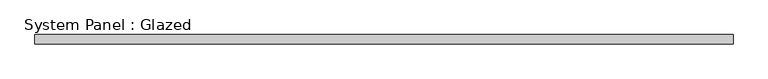
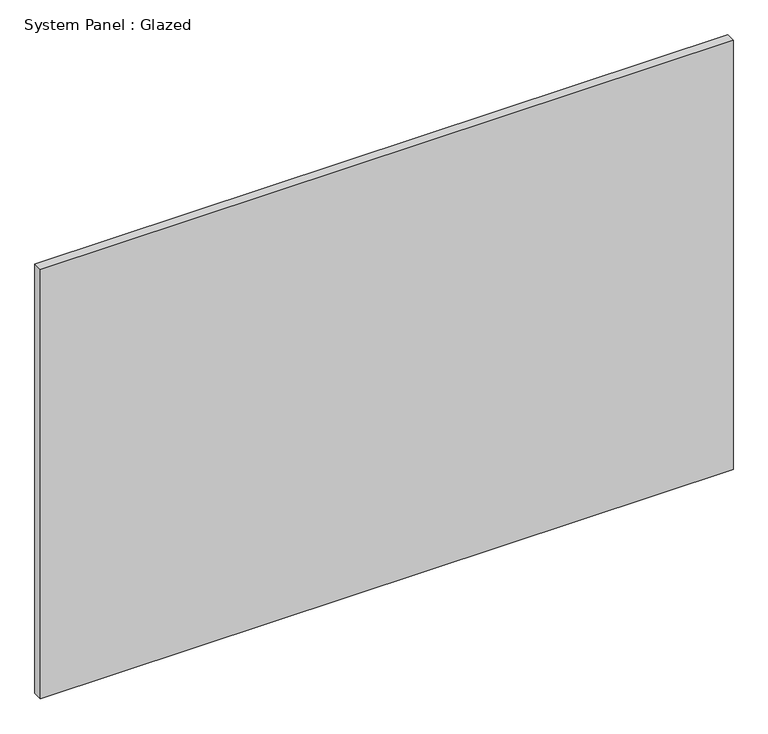
"""IFC4 building model written with IfcOpenShell, lengths in millimetres: plate geometry, System Panel : Glazed."""

from ifc_helpers import new_model, si_unit, origin, origin_with_axes, place, context, project, spatial, polyline, outline, extrude, source, transform, mapped, element, save


def system_panel_glazed_09fbcc53(model_context):
    return source(origin(), model_context, "Body", "SweptSolid", [
        extrude(outline(polyline([(915.0000002, 24.5), (-915.0000002, 24.5), (-915.0000002, 49.5), (915.0000002, 49.5), (915.0000002, 24.5)])), origin_with_axes(), (0.0, 0.0, 1.0), 1200.0),
    ])


if __name__ == "__main__":
    model = new_model("IFC4")
    model_context = context("Model", 3, world=origin())
    ifc_project = project(units=[si_unit("LENGTHUNIT", "METRE", prefix="MILLI")], contexts=[model_context])
    site = spatial("IfcSite", under=ifc_project)
    building = spatial("IfcBuilding", under=site)
    placement = place(None, origin())
    system_panel_glazed_shape = system_panel_glazed_09fbcc53(model_context)
    element("IfcPlate", 1, ObjectType="System Panel : Glazed", at=placement, inside=building, context=model_context, shape_type="MappedRepresentation", body=[
        mapped(system_panel_glazed_shape, transform((0.0, 0.0, 0.0), x_axis=(1.0, 0.0, 0.0), y_axis=(0.0, 1.0, 0.0), z_axis=(0.0, 0.0, 1.0))),
    ])
    save(model, "model.ifc")

# Revit data of these elements
# Element 1 (IfcPlate, "System Panel : Glazed")
#   Materials on its faces: "Glass"
# Materials
#   "Glass": class "Glass", colour RGB 218 227 224, transparency 0.85, Description = "Soda Lime Glass", Cost = 0
